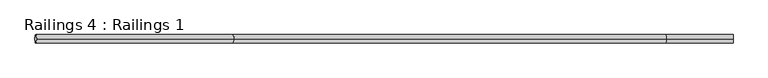
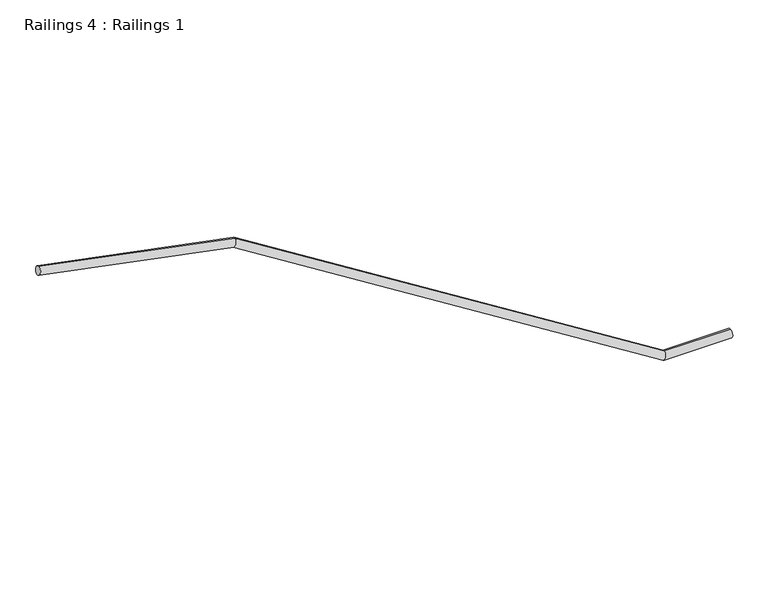
"""IFC4 building model written with IfcOpenShell, lengths in millimetres: railing geometry, Railings 4 : Railings 1."""

from ifc_helpers import new_model, si_unit, frame, origin, place, context, project, spatial, circle_curve, ellipse_curve, source, transform, mapped, element, save
from ifc_brep_helpers import plane_surface, cylinder_surface, advanced_brep


def railings_4_railings_1_2137ee24(model_context):
    return source(origin(), model_context, "Body", "AdvancedBrep", [
        advanced_brep(
        [(27446.856657, 27742.2156612, 267239.75), (27446.856657, 27742.2156612, 267277.85), (24293.568793, 27742.2156612, 268643.4603729), (24300.9445209, 27742.2156612, 268680.8396271), (27136.5721504, 27742.2156612, 267239.75), (27147.5411635, 27742.2156612, 267277.85), (25179.1116239, 27742.2156612, 268468.7237965), (25193.40169, 27742.2156612, 268504.7387035)],
        [
            (0, 1, circle_curve(frame((27446.856657, 27742.2156612, 267258.8), z_axis=(1.0, 0.0, 0.0), x_axis=(0.0, 0.0, 1.0)), 19.05)),
            (1, 0, circle_curve(frame((27446.856657, 27742.2156612, 267258.8), z_axis=(1.0, 0.0, 0.0), x_axis=(0.0, 0.0, 1.0)), 19.05)),
            (2, 3, circle_curve(frame((24297.256657, 27742.2156612, 268662.15), z_axis=(-0.9810827854808759, 0.0, 0.19358865677793646), x_axis=(0.19358865677793646, 0.0, 0.9810827854808759)), 19.05)),
            (3, 2, circle_curve(frame((24297.256657, 27742.2156612, 268662.15), z_axis=(-0.9810827854808759, 0.0, 0.19358865677793646), x_axis=(0.19358865677793646, 0.0, 0.9810827854808759)), 19.05)),
            (0, 4),
            (4, 5, ellipse_curve(frame((27142.056657, 27742.2156612, 267258.8), z_axis=(0.9609670094755092, 0.0, -0.2766629839709254), x_axis=(0.2766629839709259, 0.0, 0.9609670094755091)), 19.8237815, 19.05)),
            (5, 1),
            (5, 4, ellipse_curve(frame((27142.056657, 27742.2156612, 267258.8), z_axis=(0.9609670094755092, 0.0, -0.2766629839709254), x_axis=(0.2766629839709259, 0.0, 0.9609670094755091)), 19.8237815, 19.05)),
            (4, 6),
            (6, 7, ellipse_curve(frame((25186.256657, 27742.2156612, 268486.73125), z_axis=(0.9295045456891711, 0.0, -0.36881065540893443), x_axis=(-0.3688106554089346, 0.0, -0.929504545689171)), 19.3731742, 19.05)),
            (7, 5),
            (7, 6, ellipse_curve(frame((25186.256657, 27742.2156612, 268486.73125), z_axis=(0.9295045456891711, 0.0, -0.36881065540893443), x_axis=(-0.3688106554089346, 0.0, -0.929504545689171)), 19.3731742, 19.05)),
            (6, 2),
            (3, 7),
        ],
        [
            plane_surface(frame((27446.856657, 27723.1656612, 267258.8), z_axis=(1.0, 0.0, 0.0), x_axis=(0.0, -1.0, 0.0))),
            plane_surface(frame((24297.256657, 27723.1656612, 268662.15), z_axis=(-0.981082785480876, 0.0, 0.1935886567779364), x_axis=(0.0, -1.0, 0.0))),
            cylinder_surface(frame((27446.856657, 27742.2156612, 267258.8), z_axis=(1.0, 0.0, 0.0), x_axis=(0.0, 0.0, 1.0)), 19.05),
            cylinder_surface(frame((27142.056657, 27742.2156612, 267258.8), z_axis=(0.8469151866006068, 0.0, -0.531728000678222), x_axis=(0.531728000678222, 0.0, 0.8469151866006068)), 19.05),
            cylinder_surface(frame((25186.256657, 27742.2156612, 268486.73125), z_axis=(0.9810827854808759, 0.0, -0.19358865677793646), x_axis=(0.19358865677793646, 0.0, 0.9810827854808759)), 19.05),
        ],
        [
            (0, [[1, 2]]),
            (1, [[3, 4]]),
            (2, [[-1, 5, 6, 7]]),
            (2, [[-2, -7, 8, -5]]),
            (3, [[-6, 9, 10, 11]]),
            (3, [[-8, -11, 12, -9]]),
            (4, [[-10, 13, -4, 14]]),
            (4, [[-12, -14, -3, -13]]),
        ],
    ),
    ])


if __name__ == "__main__":
    model = new_model("IFC4")
    model_context = context("Model", 3, world=origin())
    ifc_project = project(units=[si_unit("LENGTHUNIT", "METRE", prefix="MILLI")], contexts=[model_context])
    site = spatial("IfcSite", under=ifc_project)
    building = spatial("IfcBuilding", under=site)
    placement = place(None, origin())
    railings_4_railings_1_shape = railings_4_railings_1_2137ee24(model_context)
    element("IfcRailing", 1, ObjectType="Railings 4 : Railings 1", at=placement, inside=building, context=model_context, shape_type="MappedRepresentation", body=[
        mapped(railings_4_railings_1_shape, transform((0.0, 0.0, 0.0), x_axis=(1.0, 0.0, 0.0), y_axis=(0.0, 1.0, 0.0), z_axis=(0.0, 0.0, 1.0))),
    ])
    save(model, "model.ifc")

# Revit data of these elements
# Element 1 (IfcRailing, "Railings 4 : Railings 1")
#   Materials on its faces: "ALUM. RAILING"
# Materials
#   "ALUM. RAILING": class "Generic", colour RGB 255 255 255, transparency 0, Cost = 0
